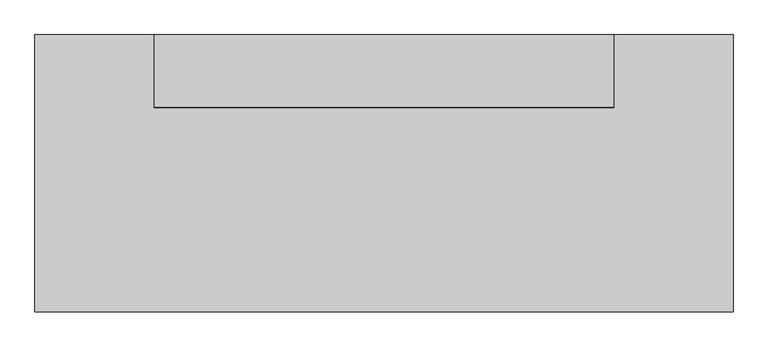
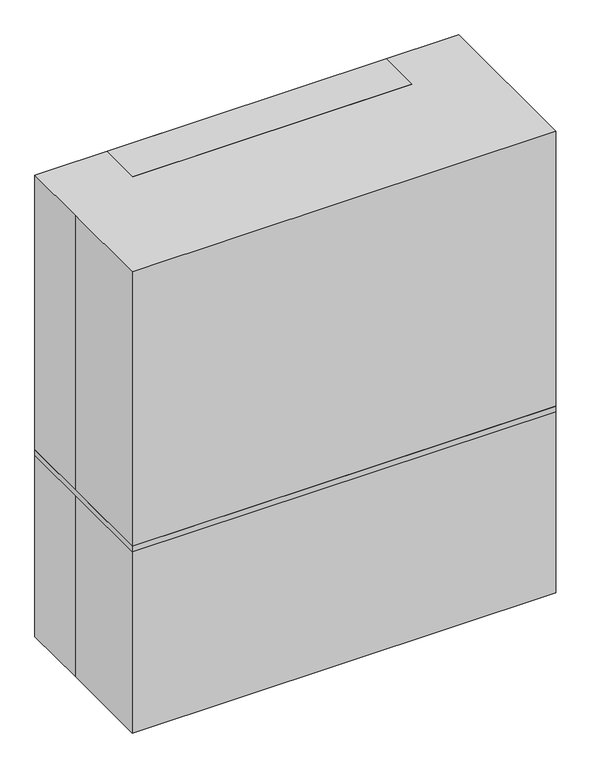
"""IFC4 building model written with IfcOpenShell, lengths in millimetres: proxy geometry, D0930 - Workstation, Dental Lab, Casting : D0930 - Workstation, Dental Lab, Casting."""

import ifcopenshell
import ifcopenshell.guid

model = None  # the IFC model being written
_history = None  # IfcOwnerHistory: only IFC2X3 demands one
_inside = {}  # id of a spatial element -> (the spatial element, [elements in it])
_under = {}  # id of a project, library or spatial element -> (it, [spatial elements below it])
_declared = {}  # id of a project -> (the project, [libraries it declares])
_typed = {}  # id of a type object -> (the type object, [elements of that type])
_made_of = {}  # id of a material, layer set ... -> (it, [elements and type objects made of it])


def new_model(schema):
    """Start an empty IFC model of exactly this schema.

    Asked for "IFC4X3", IfcOpenShell would pick the latest addendum, in which some entities
    have other attributes; the version numbers below select the first issue.
    IFC2X3 requires an IfcOwnerHistory on every rooted entity: one is made here for all.
    """
    global model, _history
    if schema == "IFC4X3":
        model = ifcopenshell.file(schema_version=(4, 3, 0, 0))
    else:
        model = ifcopenshell.file(schema=schema)
    _inside.clear()
    _under.clear()
    _declared.clear()
    _typed.clear()
    _made_of.clear()
    _history = None
    if model.schema == "IFC2X3":
        org = make("IfcOrganization", Name="unknown")
        user = make(
            "IfcPersonAndOrganization",
            ThePerson=make("IfcPerson", FamilyName="unknown"),
            TheOrganization=org,
        )
        app = make(
            "IfcApplication",
            ApplicationDeveloper=org,
            Version="unknown",
            ApplicationFullName="unknown",
            ApplicationIdentifier="unknown",
        )
        _history = make(
            "IfcOwnerHistory",
            OwningUser=user,
            OwningApplication=app,
            ChangeAction="ADDED",
            CreationDate=0,
        )
    return model


def make(cls, **values):
    """One entity of the class cls with the attributes given. An attribute that is None is left unset."""
    return model.create_entity(
        cls, **{name: value for name, value in values.items() if value is not None}
    )


def rooted(cls, **values):
    """An entity with a GlobalId (a new one), such as an element, a storey or a relation."""
    return make(cls, GlobalId=ifcopenshell.guid.new(), OwnerHistory=_history, **values)


def si_unit(unit_type, name, prefix=None):
    """IfcSIUnit, for example si_unit("LENGTHUNIT", "METRE", prefix="MILLI")."""
    return make("IfcSIUnit", UnitType=unit_type, Prefix=prefix, Name=name)


def assignment(units):
    """IfcUnitAssignment: the units of a project."""
    return None if units is None else make("IfcUnitAssignment", Units=units)


def point(xyz):
    """IfcCartesianPoint."""
    return None if xyz is None else make("IfcCartesianPoint", Coordinates=xyz)


def direction(xyz):
    """IfcDirection."""
    return None if xyz is None else make("IfcDirection", DirectionRatios=xyz)


def frame(location, z_axis=None, x_axis=None):
    """IfcAxis2Placement3D, a coordinate frame: its origin and axes. An axis left out is left unset."""
    return make(
        "IfcAxis2Placement3D",
        Location=point(location),
        Axis=direction(z_axis),
        RefDirection=direction(x_axis),
    )


def origin():
    """The frame at (0, 0, 0) with its axes left unset."""
    return frame((0.0, 0.0, 0.0))


def origin_with_axes():
    """The frame at (0, 0, 0) with the z axis (0, 0, 1) and the x axis (1, 0, 0) written out."""
    return frame((0.0, 0.0, 0.0), z_axis=(0.0, 0.0, 1.0), x_axis=(1.0, 0.0, 0.0))


def place(relative_to, where):
    """IfcLocalPlacement: puts the frame where relative to a parent placement (None: the world)."""
    return make(
        "IfcLocalPlacement", PlacementRelTo=relative_to, RelativePlacement=where
    )


def context(
    kind, dimensions, precision=None, world=None, true_north=None, identifier=None
):
    """IfcGeometricRepresentationContext, for example the 3D "Model" context."""
    return make(
        "IfcGeometricRepresentationContext",
        ContextIdentifier=identifier,
        ContextType=kind,
        CoordinateSpaceDimension=dimensions,
        Precision=precision,
        WorldCoordinateSystem=world,
        TrueNorth=true_north,
    )


def project(units=None, contexts=None):
    """IfcProject with its units and contexts."""
    return rooted(
        "IfcProject",
        Name="project",
        RepresentationContexts=contexts,
        UnitsInContext=assignment(units),
    )


def spatial(cls, under=None, at=None, **own):
    """A site, building, storey or space (cls), placed at a placement, below another one or the project."""
    s = rooted(cls, ObjectPlacement=at, **own)
    if under is not None:
        _under.setdefault(under.id(), (under, []))[1].append(s)
    return s


def polyline(points):
    """IfcPolyline through the points."""
    return make("IfcPolyline", Points=[point(p) for p in points])


def outline(outer, holes=None, kind="AREA"):
    """IfcArbitraryClosedProfileDef: a profile drawn as a closed curve; with holes, ...WithVoids."""
    if holes is None:
        return make("IfcArbitraryClosedProfileDef", ProfileType=kind, OuterCurve=outer)
    return make(
        "IfcArbitraryProfileDefWithVoids",
        ProfileType=kind,
        OuterCurve=outer,
        InnerCurves=holes,
    )


def extrude(swept, where, along, depth):
    """IfcExtrudedAreaSolid: the profile swept, set in the frame where, extruded along a direction by depth."""
    return make(
        "IfcExtrudedAreaSolid",
        SweptArea=swept,
        Position=where,
        ExtrudedDirection=direction(along),
        Depth=depth,
    )


def shape(context_of_items, identifier, shape_type, items):
    """IfcShapeRepresentation: the items that make up one representation, for example the "Body"."""
    return make(
        "IfcShapeRepresentation",
        ContextOfItems=context_of_items,
        RepresentationIdentifier=identifier,
        RepresentationType=shape_type,
        Items=items,
    )


def source(mapping_origin, context_of_items, identifier, shape_type, items):
    """IfcRepresentationMap: a shape defined once, which mapped items show again and again."""
    return make(
        "IfcRepresentationMap",
        MappingOrigin=mapping_origin,
        MappedRepresentation=shape(context_of_items, identifier, shape_type, items),
    )


def transform(
    local_origin,
    x_axis=None,
    y_axis=None,
    z_axis=None,
    scale=None,
    scale2=None,
    scale3=None,
    uniform=True,
):
    """IfcCartesianTransformationOperator3D, or its non-uniform kind. x_axis, y_axis, z_axis: its Axis1, 2, 3."""
    if uniform:
        return make(
            "IfcCartesianTransformationOperator3D",
            Axis1=direction(x_axis),
            Axis2=direction(y_axis),
            LocalOrigin=point(local_origin),
            Scale=scale,
            Axis3=direction(z_axis),
        )
    return make(
        "IfcCartesianTransformationOperator3DnonUniform",
        Axis1=direction(x_axis),
        Axis2=direction(y_axis),
        LocalOrigin=point(local_origin),
        Scale=scale,
        Axis3=direction(z_axis),
        Scale2=scale2,
        Scale3=scale3,
    )


def mapped(mapping_source, mapping_target):
    """IfcMappedItem: shows the shape of a source again, moved by a transform."""
    return make(
        "IfcMappedItem", MappingSource=mapping_source, MappingTarget=mapping_target
    )


def made_of(thing, what):
    """Note that an element or type object is made of a material, layer set ...; save() writes the relation."""
    if what is not None:
        _made_of.setdefault(what.id(), (what, []))[1].append(thing)
    return thing


def element(
    cls,
    number,
    at=None,
    inside=None,
    cuts=None,
    type_object=None,
    material=None,
    context=None,
    identifier="Body",
    shape_type=None,
    held_by="IfcProductDefinitionShape",
    body=None,
    shapes=None,
    **own,
):
    """One element of the class cls, such as IfcWall. Its Tag is "e" and its number.

    at: its placement. inside: the storey or other place that contains it. cuts: it is an
    opening in that element (IfcRelVoidsElement). A single representation is given by context,
    identifier, shape_type and body (its items); several are given by shapes. held_by: the class
    of the entity that holds the representations. save() writes the other relations.
    """
    e = rooted(cls, Tag="e%d" % number, ObjectPlacement=at, **own)
    if body is not None:
        shapes = [shape(context, identifier, shape_type, body)]
    if shapes is not None:
        e.Representation = make(held_by, Representations=shapes)
    if inside is not None:
        _inside.setdefault(inside.id(), (inside, []))[1].append(e)
    if cuts is not None:
        rooted(
            "IfcRelVoidsElement", RelatingBuildingElement=cuts, RelatedOpeningElement=e
        )
    if type_object is not None:
        _typed.setdefault(type_object.id(), (type_object, []))[1].append(e)
    return made_of(e, material)


def aggregate(whole, parts):
    """IfcRelAggregates: a whole, such as a stair, and the parts it consists of."""
    return rooted("IfcRelAggregates", RelatingObject=whole, RelatedObjects=parts)


def save(model, path):
    """Write the relations noted so far, then the file.

    IfcRelAggregates (storeys below a building ...), IfcRelContainedInSpatialStructure (elements
    in a storey), IfcRelDefinesByType, IfcRelAssociatesMaterial and IfcRelDeclares: one each for
    every whole, place, type object, material and project.
    """
    for whole, parts in _under.values():
        aggregate(whole, parts)
    for where, things in _inside.values():
        rooted(
            "IfcRelContainedInSpatialStructure",
            RelatedElements=things,
            RelatingStructure=where,
        )
    for kind, things in _typed.values():
        rooted("IfcRelDefinesByType", RelatedObjects=things, RelatingType=kind)
    for what, things in _made_of.values():
        rooted("IfcRelAssociatesMaterial", RelatedObjects=things, RelatingMaterial=what)
    for by, libraries in _declared.values():
        rooted("IfcRelDeclares", RelatingContext=by, RelatedDefinitions=libraries)
    model.write(path)


def specialty_equipment_0b9d7219(model_context):
    return source(origin(), model_context, "Body", "SweptSolid", [
        extrude(outline(polyline([(-609.6, 342.9), (-609.6, 368.3), (-558.8, 368.3), (-558.8, 342.9), (-609.6, 342.9)])), frame((0.0, 0.0, 1524.0), z_axis=(0.0, 0.0, 1.0), x_axis=(1.0, 0.0, 0.0)), (0.0, 0.0, 1.0), 406.4),
        extrude(outline(polyline([(609.6, 368.3), (609.6, 342.9), (558.8, 342.9), (558.8, 368.3), (609.6, 368.3)])), frame((0.0, 0.0, 1524.0), z_axis=(0.0, 0.0, 1.0), x_axis=(1.0, 0.0, 0.0)), (0.0, 0.0, 1.0), 406.4),
        extrude(outline(polyline([(609.6, -88.9), (-609.6, -88.9), (-609.6, 368.3), (609.6, 368.3), (609.6, -88.9)])), frame((0.0, 0.0, 1498.6), z_axis=(0.0, 0.0, 1.0), x_axis=(1.0, 0.0, 0.0)), (0.0, 0.0, 1.0), 25.4),
        extrude(outline(polyline([(175.0645431, 2133.6), (368.3, 2133.6), (368.3, 1930.4), (-88.9, 1930.4), (-88.9, 1981.2), (175.0645431, 2133.6)])), frame((-609.6, 0.0, 0.0), z_axis=(1.0, 0.0, 0.0), x_axis=(0.0, 1.0, 0.0)), (0.0, 0.0, 1.0), 1219.2),
        extrude(outline(polyline([(-901.7, -342.9), (-901.7, 342.9), (901.7, 342.9), (901.7, -342.9), (889.0, -342.9), (889.0, 330.2), (-889.0, 330.2), (-889.0, -342.9), (-901.7, -342.9)])), origin_with_axes(), (0.0, 0.0, 1.0), 838.2),
        extrude(outline(polyline([(927.1, 368.3), (927.1, -368.3), (-927.1, -368.3), (-927.1, 368.3), (927.1, 368.3)])), frame((0.0, 0.0, 838.2), z_axis=(0.0, 0.0, 1.0), x_axis=(1.0, 0.0, 0.0)), (0.0, 0.0, 1.0), 25.4),
        extrude(outline(polyline([(-927.1, 368.3), (927.1, 368.3), (927.1, -368.3), (-927.1, -368.3), (-927.1, 63.5), (-927.1, 368.3)])), origin_with_axes(), (0.0, 0.0, 1.0), 2133.6),
    ])


if __name__ == "__main__":
    model = new_model("IFC4")
    model_context = context("Model", 3, world=origin())
    ifc_project = project(units=[si_unit("LENGTHUNIT", "METRE", prefix="MILLI")], contexts=[model_context])
    site = spatial("IfcSite", under=ifc_project)
    building = spatial("IfcBuilding", under=site)
    placement = place(None, origin())
    specialty_equipment_shape = specialty_equipment_0b9d7219(model_context)
    element("IfcBuildingElementProxy", 1, Name="D0930 - Workstation, Dental Lab, Casting : D0930 - Workstation, Dental Lab, Casting", ObjectType="D0930 - Workstation, Dental Lab, Casting : D0930 - Workstation, Dental Lab, Casting", at=placement, inside=building, context=model_context, shape_type="MappedRepresentation", body=[
        mapped(specialty_equipment_shape, transform((0.0, 0.0, 0.0), x_axis=(1.0, 0.0, 0.0), y_axis=(0.0, 1.0, 0.0), z_axis=(0.0, 0.0, 1.0))),
    ])
    save(model, "model.ifc")

# Revit data of these elements
# Type "D0930 - Workstation, Dental Lab, Casting : D0930 - Workstation, Dental Lab, Casting"
#   Watts2 = "0"
#   Watts1 = "1200"
#   Unit_Issue = "EA"
#   UTIL_6_Misc = "E"
#   UTIL_5_NonMedGas = "-"
#   UTIL_4_MiscGas = "-"
#   UTIL_3_MedGas = "-"
#   UTIL_2_Elec = "A"
#   UTIL_1_WaterDrain = "-"
#   Nomenclature = "Workstation, Dental Lab, Casting"
#   NSN = "6520"
#   Location [instance default] = ""
#   JSN = "D0930"
#   Fund_Source_VA = "-"
#   Fund_Source_Navy = "A"
#   Fund_Source_Army = "A"
#   Fund_Source_AF = "A"
#   ELEC_Volts2 = "0"
#   ELEC_Volts1 = "120"
#   ELEC_Phase2 = "0"
#   ELEC_Phase1 = "1"
#   ELEC_HertzSwitch = "0"
#   ELEC_HertzDependent = "-1"
#   ELEC_Hertz = "60"
#   ELEC_Amps2 = "0"
#   ELEC_Amps1 = "10"
#   DetailDescription = "Modular casting workstation which includes a full-length load-bearing aluminum frame on adjustable legs with side panels and supports, an overhead stainless steel ventilation canopy hood (options include a start delay and 99 hour timer), a furnace shelf (48\"Lx16\"D), a pullout casting ring cooling drawer with steel grid and a ceramic tile countertop."
#   CAT_VA = "A"
#   CAT_Navy = "A"
#   CAT_IHS = "-"
#   CAT_Army = "A"
#   CAT_AF = "A"
#   BTUperhour = "0"
#   Weight_IP = 675
#   DIM_Width_IP = 6' - 1"
#   DIM_Height_IP = 7' - 0"
#   DIM_Depth_IP = 2' - 5"
# Element 1 (IfcBuildingElementProxy, "D0930 - Workstation, Dental Lab, Casting : D0930 - Workstation, Dental Lab, Casting")
#   Location = "DNPL2"
#   Materials on its faces: "EquipSpace"
# Materials
#   "EquipSpace": class "Unassigned", colour RGB 221 217 195, transparency 0.5
